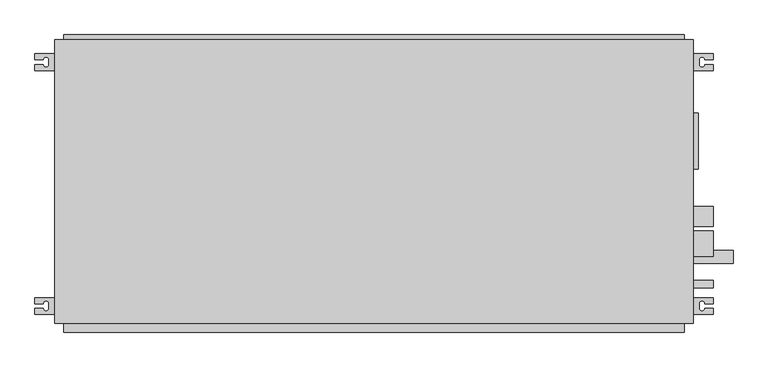
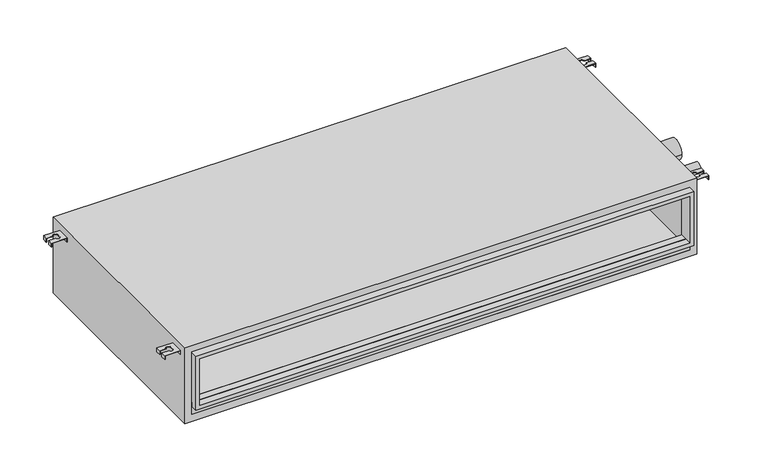
"""IFC4 building model written with IfcOpenShell, lengths in millimetres: proxy geometry, PEFY-P-NMAU-E_Medium_Static_Ducted : PEFY-P54NMAU-E."""

import ifcopenshell
import ifcopenshell.guid

model = None  # the IFC model being written
_history = None  # IfcOwnerHistory: only IFC2X3 demands one
_inside = {}  # id of a spatial element -> (the spatial element, [elements in it])
_under = {}  # id of a project, library or spatial element -> (it, [spatial elements below it])
_declared = {}  # id of a project -> (the project, [libraries it declares])
_typed = {}  # id of a type object -> (the type object, [elements of that type])
_made_of = {}  # id of a material, layer set ... -> (it, [elements and type objects made of it])


def new_model(schema):
    """Start an empty IFC model of exactly this schema.

    Asked for "IFC4X3", IfcOpenShell would pick the latest addendum, in which some entities
    have other attributes; the version numbers below select the first issue.
    IFC2X3 requires an IfcOwnerHistory on every rooted entity: one is made here for all.
    """
    global model, _history
    if schema == "IFC4X3":
        model = ifcopenshell.file(schema_version=(4, 3, 0, 0))
    else:
        model = ifcopenshell.file(schema=schema)
    _inside.clear()
    _under.clear()
    _declared.clear()
    _typed.clear()
    _made_of.clear()
    _history = None
    if model.schema == "IFC2X3":
        org = make("IfcOrganization", Name="unknown")
        user = make(
            "IfcPersonAndOrganization",
            ThePerson=make("IfcPerson", FamilyName="unknown"),
            TheOrganization=org,
        )
        app = make(
            "IfcApplication",
            ApplicationDeveloper=org,
            Version="unknown",
            ApplicationFullName="unknown",
            ApplicationIdentifier="unknown",
        )
        _history = make(
            "IfcOwnerHistory",
            OwningUser=user,
            OwningApplication=app,
            ChangeAction="ADDED",
            CreationDate=0,
        )
    return model


def make(cls, **values):
    """One entity of the class cls with the attributes given. An attribute that is None is left unset."""
    return model.create_entity(
        cls, **{name: value for name, value in values.items() if value is not None}
    )


def rooted(cls, **values):
    """An entity with a GlobalId (a new one), such as an element, a storey or a relation."""
    return make(cls, GlobalId=ifcopenshell.guid.new(), OwnerHistory=_history, **values)


def si_unit(unit_type, name, prefix=None):
    """IfcSIUnit, for example si_unit("LENGTHUNIT", "METRE", prefix="MILLI")."""
    return make("IfcSIUnit", UnitType=unit_type, Prefix=prefix, Name=name)


def assignment(units):
    """IfcUnitAssignment: the units of a project."""
    return None if units is None else make("IfcUnitAssignment", Units=units)


def point(xyz):
    """IfcCartesianPoint."""
    return None if xyz is None else make("IfcCartesianPoint", Coordinates=xyz)


def direction(xyz):
    """IfcDirection."""
    return None if xyz is None else make("IfcDirection", DirectionRatios=xyz)


def frame(location, z_axis=None, x_axis=None):
    """IfcAxis2Placement3D, a coordinate frame: its origin and axes. An axis left out is left unset."""
    return make(
        "IfcAxis2Placement3D",
        Location=point(location),
        Axis=direction(z_axis),
        RefDirection=direction(x_axis),
    )


def frame_2d(location, x_axis=None):
    """IfcAxis2Placement2D, a coordinate frame in the plane: its origin and x axis."""
    return make(
        "IfcAxis2Placement2D", Location=point(location), RefDirection=direction(x_axis)
    )


def origin():
    """The frame at (0, 0, 0) with its axes left unset."""
    return frame((0.0, 0.0, 0.0))


def place(relative_to, where):
    """IfcLocalPlacement: puts the frame where relative to a parent placement (None: the world)."""
    return make(
        "IfcLocalPlacement", PlacementRelTo=relative_to, RelativePlacement=where
    )


def context(
    kind, dimensions, precision=None, world=None, true_north=None, identifier=None
):
    """IfcGeometricRepresentationContext, for example the 3D "Model" context."""
    return make(
        "IfcGeometricRepresentationContext",
        ContextIdentifier=identifier,
        ContextType=kind,
        CoordinateSpaceDimension=dimensions,
        Precision=precision,
        WorldCoordinateSystem=world,
        TrueNorth=true_north,
    )


def project(units=None, contexts=None):
    """IfcProject with its units and contexts."""
    return rooted(
        "IfcProject",
        Name="project",
        RepresentationContexts=contexts,
        UnitsInContext=assignment(units),
    )


def spatial(cls, under=None, at=None, **own):
    """A site, building, storey or space (cls), placed at a placement, below another one or the project."""
    s = rooted(cls, ObjectPlacement=at, **own)
    if under is not None:
        _under.setdefault(under.id(), (under, []))[1].append(s)
    return s


def polyline(points):
    """IfcPolyline through the points."""
    return make("IfcPolyline", Points=[point(p) for p in points])


def circle_curve(where, radius):
    """IfcCircle in the frame where."""
    return make("IfcCircle", Position=where, Radius=radius)


def trimmed(basis, trim1, trim2, sense, master):
    """IfcTrimmedCurve: the piece of a basis curve between two trims."""
    return make(
        "IfcTrimmedCurve",
        BasisCurve=basis,
        Trim1=trim1,
        Trim2=trim2,
        SenseAgreement=sense,
        MasterRepresentation=master,
    )


def segment(curve, same_sense, transition):
    """IfcCompositeCurveSegment."""
    return make(
        "IfcCompositeCurveSegment",
        Transition=transition,
        SameSense=same_sense,
        ParentCurve=curve,
    )


def composite_curve(segments, self_intersect=None):
    """IfcCompositeCurve: segments joined end to end."""
    return make("IfcCompositeCurve", Segments=segments, SelfIntersect=self_intersect)


def outline(outer, holes=None, kind="AREA"):
    """IfcArbitraryClosedProfileDef: a profile drawn as a closed curve; with holes, ...WithVoids."""
    if holes is None:
        return make("IfcArbitraryClosedProfileDef", ProfileType=kind, OuterCurve=outer)
    return make(
        "IfcArbitraryProfileDefWithVoids",
        ProfileType=kind,
        OuterCurve=outer,
        InnerCurves=holes,
    )


def extrude(swept, where, along, depth):
    """IfcExtrudedAreaSolid: the profile swept, set in the frame where, extruded along a direction by depth."""
    return make(
        "IfcExtrudedAreaSolid",
        SweptArea=swept,
        Position=where,
        ExtrudedDirection=direction(along),
        Depth=depth,
    )


def shape(context_of_items, identifier, shape_type, items):
    """IfcShapeRepresentation: the items that make up one representation, for example the "Body"."""
    return make(
        "IfcShapeRepresentation",
        ContextOfItems=context_of_items,
        RepresentationIdentifier=identifier,
        RepresentationType=shape_type,
        Items=items,
    )


def source(mapping_origin, context_of_items, identifier, shape_type, items):
    """IfcRepresentationMap: a shape defined once, which mapped items show again and again."""
    return make(
        "IfcRepresentationMap",
        MappingOrigin=mapping_origin,
        MappedRepresentation=shape(context_of_items, identifier, shape_type, items),
    )


def transform(
    local_origin,
    x_axis=None,
    y_axis=None,
    z_axis=None,
    scale=None,
    scale2=None,
    scale3=None,
    uniform=True,
):
    """IfcCartesianTransformationOperator3D, or its non-uniform kind. x_axis, y_axis, z_axis: its Axis1, 2, 3."""
    if uniform:
        return make(
            "IfcCartesianTransformationOperator3D",
            Axis1=direction(x_axis),
            Axis2=direction(y_axis),
            LocalOrigin=point(local_origin),
            Scale=scale,
            Axis3=direction(z_axis),
        )
    return make(
        "IfcCartesianTransformationOperator3DnonUniform",
        Axis1=direction(x_axis),
        Axis2=direction(y_axis),
        LocalOrigin=point(local_origin),
        Scale=scale,
        Axis3=direction(z_axis),
        Scale2=scale2,
        Scale3=scale3,
    )


def mapped(mapping_source, mapping_target):
    """IfcMappedItem: shows the shape of a source again, moved by a transform."""
    return make(
        "IfcMappedItem", MappingSource=mapping_source, MappingTarget=mapping_target
    )


def made_of(thing, what):
    """Note that an element or type object is made of a material, layer set ...; save() writes the relation."""
    if what is not None:
        _made_of.setdefault(what.id(), (what, []))[1].append(thing)
    return thing


def element(
    cls,
    number,
    at=None,
    inside=None,
    cuts=None,
    type_object=None,
    material=None,
    context=None,
    identifier="Body",
    shape_type=None,
    held_by="IfcProductDefinitionShape",
    body=None,
    shapes=None,
    **own,
):
    """One element of the class cls, such as IfcWall. Its Tag is "e" and its number.

    at: its placement. inside: the storey or other place that contains it. cuts: it is an
    opening in that element (IfcRelVoidsElement). A single representation is given by context,
    identifier, shape_type and body (its items); several are given by shapes. held_by: the class
    of the entity that holds the representations. save() writes the other relations.
    """
    e = rooted(cls, Tag="e%d" % number, ObjectPlacement=at, **own)
    if body is not None:
        shapes = [shape(context, identifier, shape_type, body)]
    if shapes is not None:
        e.Representation = make(held_by, Representations=shapes)
    if inside is not None:
        _inside.setdefault(inside.id(), (inside, []))[1].append(e)
    if cuts is not None:
        rooted(
            "IfcRelVoidsElement", RelatingBuildingElement=cuts, RelatedOpeningElement=e
        )
    if type_object is not None:
        _typed.setdefault(type_object.id(), (type_object, []))[1].append(e)
    return made_of(e, material)


def aggregate(whole, parts):
    """IfcRelAggregates: a whole, such as a stair, and the parts it consists of."""
    return rooted("IfcRelAggregates", RelatingObject=whole, RelatedObjects=parts)


def save(model, path):
    """Write the relations noted so far, then the file.

    IfcRelAggregates (storeys below a building ...), IfcRelContainedInSpatialStructure (elements
    in a storey), IfcRelDefinesByType, IfcRelAssociatesMaterial and IfcRelDeclares: one each for
    every whole, place, type object, material and project.
    """
    for whole, parts in _under.values():
        aggregate(whole, parts)
    for where, things in _inside.values():
        rooted(
            "IfcRelContainedInSpatialStructure",
            RelatedElements=things,
            RelatingStructure=where,
        )
    for kind, things in _typed.values():
        rooted("IfcRelDefinesByType", RelatedObjects=things, RelatingType=kind)
    for what, things in _made_of.values():
        rooted("IfcRelAssociatesMaterial", RelatedObjects=things, RelatingMaterial=what)
    for by, libraries in _declared.values():
        rooted("IfcRelDeclares", RelatingContext=by, RelatedDefinitions=libraries)
    model.write(path)


def plane_surface(at):
    """IfcPlane: the flat surface through the origin of the frame at, square to its z axis."""
    return make("IfcPlane", Position=at)


def revolved_surface(curve, axis_point, axis_direction):
    """IfcSurfaceOfRevolution: the curve turned about the line through axis_point along axis_direction."""
    return make(
        "IfcSurfaceOfRevolution",
        SweptCurve=make("IfcArbitraryOpenProfileDef", ProfileType="CURVE", Curve=curve),
        AxisPosition=make("IfcAxis1Placement", Location=point(axis_point), Axis=direction(axis_direction)),
    )


def advanced_brep(points, edges, surfaces, faces):
    """IfcAdvancedBrep: a solid bounded by faces that lie on surfaces and meet in shared edges.

    An edge is (start, end): straight between two places in points (the first is 0);
    or (start, end, curve); or (start, end, curve, False) where it runs against its curve.
    A face is (place in surfaces, loops), or (place, loops, False) where it looks against
    its surface's normal. A loop lists edges by number (the first is 1), with a minus sign
    where the edge is run from its end to its start. The first loop is the outer one.
    """
    corners = [point(p) for p in points]
    vertices = [make("IfcVertexPoint", VertexGeometry=c) for c in corners]
    made = []
    for start, end, *more in edges:
        made.append(
            make(
                "IfcEdgeCurve",
                EdgeStart=vertices[start],
                EdgeEnd=vertices[end],
                EdgeGeometry=more[0] if more else make("IfcPolyline", Points=[corners[start], corners[end]]),
                SameSense=more[1] if len(more) > 1 else True,
            )
        )
    hull = []
    for where, loops, *sense in faces:
        bounds = []
        for j, loop in enumerate(loops):
            ring = [make("IfcOrientedEdge", EdgeElement=made[abs(k) - 1], Orientation=k > 0) for k in loop]
            bounds.append(
                make(
                    "IfcFaceOuterBound" if j == 0 else "IfcFaceBound",
                    Bound=make("IfcEdgeLoop", EdgeList=ring),
                    Orientation=True,
                )
            )
        hull.append(make("IfcAdvancedFace", Bounds=bounds, FaceSurface=surfaces[where], SameSense=sense[0] if sense else True))
    return make("IfcAdvancedBrep", Outer=make("IfcClosedShell", CfsFaces=hull))


def mechanical_equipment_8a2286fb(model_context):
    return source(origin(), model_context, "Body", "SolidModel", [
        advanced_brep(
        [(-860.118493, -231.05, 249.2375), (-860.118493, -246.05, 249.2375), (-839.112243, -246.05, 249.2375), (-825.112243, -246.05, 249.2375), (-825.112243, -258.05, 249.2375), (-839.112243, -258.05, 249.2375), (-860.118493, -258.05, 249.2375), (-860.118493, -273.05, 249.2375), (-810.112243, -273.05, 249.2375), (-810.112243, -231.05, 249.2375), (-860.118493, -231.05, 236.4972162), (-858.530493, -231.05, 236.4972162), (-858.530493, -246.05, 236.4972162), (-860.118493, -246.05, 236.4972162), (-858.530493, -273.05, 236.4972162), (-860.118493, -273.05, 236.4972162), (-860.118493, -258.05, 236.4972162), (-858.530493, -258.05, 236.4972162), (-810.112243, -231.05, 236.4972162), (-810.112243, -273.05, 236.4972162), (-811.700243, -273.05, 236.4972162), (-811.700243, -231.05, 236.4972162), (-858.530493, -246.05, 247.65), (-839.112243, -246.05, 247.65), (-858.530493, -231.05, 247.65), (-811.700243, -231.05, 247.65), (-858.530493, -258.05, 247.65), (-858.530493, -273.05, 247.65), (-839.112243, -258.05, 247.65), (-811.700243, -273.05, 247.65), (-825.112243, -258.05, 247.65), (-825.112243, -246.05, 247.65)],
        [
            (0, 1),
            (1, 2),
            (2, 3, circle_curve(frame((-832.112243, -246.05, 249.2375), z_axis=(0.0, 0.0, -1.0), x_axis=(1.0, 0.0, 0.0)), 7.0)),
            (3, 4),
            (4, 5, circle_curve(frame((-832.112243, -258.05, 249.2375), z_axis=(0.0, 0.0, -1.0), x_axis=(1.0, 0.0, 0.0)), 7.0)),
            (5, 6),
            (6, 7),
            (7, 8),
            (8, 9),
            (9, 0),
            (10, 11),
            (11, 12),
            (12, 13),
            (13, 10),
            (14, 15),
            (15, 16),
            (16, 17),
            (17, 14),
            (18, 19),
            (19, 20),
            (20, 21),
            (21, 18),
            (13, 1),
            (0, 10),
            (12, 22),
            (22, 23),
            (23, 2),
            (11, 24),
            (24, 22),
            (9, 18),
            (21, 25),
            (25, 24),
            (17, 26),
            (26, 27),
            (27, 14),
            (5, 28),
            (28, 26),
            (16, 6),
            (15, 7),
            (27, 29),
            (29, 20),
            (19, 8),
            (29, 25),
            (30, 31),
            (31, 23, circle_curve(frame((-832.112243, -246.05, 247.65), z_axis=(0.0, 0.0, 1.0), x_axis=(1.0, 0.0, 0.0)), 7.0)),
            (28, 30, circle_curve(frame((-832.112243, -258.05, 247.65), z_axis=(0.0, 0.0, 1.0), x_axis=(1.0, 0.0, 0.0)), 7.0)),
            (4, 30),
            (31, 3),
        ],
        [
            plane_surface(frame((-860.118493, -231.05, 249.2375), z_axis=(0.0, 0.0, 1.0), x_axis=(0.0, -1.0, 0.0))),
            plane_surface(frame((-860.118493, -231.05, 236.4972162), z_axis=(0.0, 0.0, -1.0), x_axis=(0.0, 1.0, 0.0))),
            plane_surface(frame((-860.118493, -231.05, 249.2375), z_axis=(-1.0, 0.0, 0.0), x_axis=(0.0, 0.0, -1.0))),
            plane_surface(frame((-860.118493, -246.05, 249.2375), z_axis=(0.0, -1.0, 0.0), x_axis=(0.0, 0.0, -1.0))),
            plane_surface(frame((-858.530493, -246.05, 249.2375), z_axis=(1.0, 0.0, 0.0), x_axis=(0.0, 0.0, -1.0))),
            plane_surface(frame((-858.530493, -231.05, 249.2375), z_axis=(0.0, 1.0, 0.0), x_axis=(0.0, 0.0, -1.0))),
            plane_surface(frame((-858.530493, -273.05, 249.2375), z_axis=(1.0, 0.0, 0.0), x_axis=(0.0, 0.0, -1.0))),
            plane_surface(frame((-858.530493, -258.05, 249.2375), z_axis=(0.0, 1.0, 0.0), x_axis=(0.0, 0.0, -1.0))),
            plane_surface(frame((-860.118493, -258.05, 249.2375), z_axis=(-1.0, 0.0, 0.0), x_axis=(0.0, 0.0, -1.0))),
            plane_surface(frame((-860.118493, -273.05, 249.2375), z_axis=(0.0, -1.0, 0.0), x_axis=(0.0, 0.0, -1.0))),
            plane_surface(frame((-811.700243, -231.05, 249.2375), z_axis=(-1.0, 0.0, 0.0), x_axis=(0.0, 0.0, -1.0))),
            plane_surface(frame((-810.112243, -273.05, 249.2375), z_axis=(1.0, 0.0, 0.0), x_axis=(0.0, 0.0, -1.0))),
            plane_surface(frame((-825.112243, -258.05, 247.65), z_axis=(0.0, 0.0, -1.0), x_axis=(0.0, 1.0, 0.0))),
            revolved_surface(polyline([(-825.112243, -258.05, 247.65), (-825.112243, -258.05, 249.2375)]), (-832.112243, -258.05, 247.65), (0.0, 0.0, -1.0)),
            revolved_surface(polyline([(-825.112243, -246.05, 247.65), (-825.112243, -246.05, 249.2375)]), (-832.112243, -246.05, 247.65), (0.0, 0.0, -1.0)),
            plane_surface(frame((-825.112243, -246.05, 249.2375), z_axis=(-1.0, 0.0, 0.0), x_axis=(0.0, 0.0, -1.0))),
        ],
        [
            (0, [[1, 2, 3, 4, 5, 6, 7, 8, 9, 10]]),
            (1, [[11, 12, 13, 14]]),
            (1, [[15, 16, 17, 18]]),
            (1, [[19, 20, 21, 22]]),
            (2, [[23, -1, 24, -14]]),
            (3, [[-2, -23, -13, 25, 26, 27]]),
            (4, [[-12, 28, 29, -25]]),
            (5, [[-10, 30, -22, 31, 32, -28, -11, -24]]),
            (6, [[-18, 33, 34, 35]]),
            (7, [[-6, 36, 37, -33, -17, 38]]),
            (8, [[39, -7, -38, -16]]),
            (9, [[-8, -39, -15, -35, 40, 41, -20, 42]]),
            (10, [[-21, -41, 43, -31]]),
            (11, [[-30, -9, -42, -19]]),
            (12, [[44, 45, -26, -29, -32, -43, -40, -34, -37, 46]]),
            (13, [[-5, 47, -46, -36]]),
            (14, [[-3, -27, -45, 48]]),
            (15, [[-4, -48, -44, -47]]),
        ],
    ),
        advanced_brep(
        [(840.094007, -231.05, 249.2375), (790.087757, -231.05, 249.2375), (790.087757, -273.05, 249.2375), (840.094007, -273.05, 249.2375), (840.094007, -258.05, 249.2375), (819.087757, -258.05, 249.2375), (805.087757, -258.05, 249.2375), (805.087757, -246.05, 249.2375), (819.087757, -246.05, 249.2375), (840.094007, -246.05, 249.2375), (840.094007, -231.05, 236.4972162), (840.094007, -246.05, 236.4972162), (838.506007, -246.05, 236.4972162), (838.506007, -231.05, 236.4972162), (838.506007, -273.05, 236.4972162), (838.506007, -258.05, 236.4972162), (840.094007, -258.05, 236.4972162), (840.094007, -273.05, 236.4972162), (790.087757, -231.05, 236.4972162), (791.675757, -231.05, 236.4972162), (791.675757, -273.05, 236.4972162), (790.087757, -273.05, 236.4972162), (819.087757, -246.05, 247.65), (838.506007, -246.05, 247.65), (838.506007, -231.05, 247.65), (791.675757, -231.05, 247.65), (838.506007, -273.05, 247.65), (838.506007, -258.05, 247.65), (819.087757, -258.05, 247.65), (791.675757, -273.05, 247.65), (805.087757, -258.05, 247.65), (805.087757, -246.05, 247.65)],
        [
            (0, 1),
            (1, 2),
            (2, 3),
            (3, 4),
            (4, 5),
            (5, 6, circle_curve(frame((812.087757, -258.05, 249.2375), z_axis=(0.0, 0.0, -1.0), x_axis=(-1.0, 0.0, 0.0)), 7.0)),
            (6, 7),
            (7, 8, circle_curve(frame((812.087757, -246.05, 249.2375), z_axis=(0.0, 0.0, -1.0), x_axis=(-1.0, 0.0, 0.0)), 7.0)),
            (8, 9),
            (9, 0),
            (10, 11),
            (11, 12),
            (12, 13),
            (13, 10),
            (14, 15),
            (15, 16),
            (16, 17),
            (17, 14),
            (18, 19),
            (19, 20),
            (20, 21),
            (21, 18),
            (10, 0),
            (9, 11),
            (8, 22),
            (22, 23),
            (23, 12),
            (23, 24),
            (24, 13),
            (24, 25),
            (25, 19),
            (18, 1),
            (14, 26),
            (26, 27),
            (27, 15),
            (4, 16),
            (27, 28),
            (28, 5),
            (3, 17),
            (2, 21),
            (20, 29),
            (29, 26),
            (25, 29),
            (30, 28, circle_curve(frame((812.087757, -258.05, 247.65), z_axis=(0.0, 0.0, 1.0), x_axis=(-1.0, 0.0, 0.0)), 7.0)),
            (22, 31, circle_curve(frame((812.087757, -246.05, 247.65), z_axis=(0.0, 0.0, 1.0), x_axis=(-1.0, 0.0, 0.0)), 7.0)),
            (31, 30),
            (30, 6),
            (7, 31),
        ],
        [
            plane_surface(frame((840.094007, -231.05, 249.2375), z_axis=(0.0, 0.0, 1.0), x_axis=(0.0, -1.0, 0.0))),
            plane_surface(frame((840.094007, -231.05, 236.4972162), z_axis=(0.0, 0.0, -1.0), x_axis=(0.0, 1.0, 0.0))),
            plane_surface(frame((840.094007, -231.05, 249.2375), z_axis=(1.0, 0.0, 0.0), x_axis=(0.0, 0.0, -1.0))),
            plane_surface(frame((840.094007, -246.05, 249.2375), z_axis=(0.0, -1.0, 0.0), x_axis=(0.0, 0.0, -1.0))),
            plane_surface(frame((838.506007, -246.05, 249.2375), z_axis=(-1.0, 0.0, 0.0), x_axis=(0.0, 0.0, -1.0))),
            plane_surface(frame((838.506007, -231.05, 249.2375), z_axis=(0.0, 1.0, 0.0), x_axis=(0.0, 0.0, -1.0))),
            plane_surface(frame((838.506007, -273.05, 249.2375), z_axis=(-1.0, 0.0, 0.0), x_axis=(0.0, 0.0, -1.0))),
            plane_surface(frame((838.506007, -258.05, 249.2375), z_axis=(0.0, 1.0, 0.0), x_axis=(0.0, 0.0, -1.0))),
            plane_surface(frame((840.094007, -258.05, 249.2375), z_axis=(1.0, 0.0, 0.0), x_axis=(0.0, 0.0, -1.0))),
            plane_surface(frame((840.094007, -273.05, 249.2375), z_axis=(0.0, -1.0, 0.0), x_axis=(0.0, 0.0, -1.0))),
            plane_surface(frame((791.675757, -231.05, 249.2375), z_axis=(1.0, 0.0, 0.0), x_axis=(0.0, 0.0, -1.0))),
            plane_surface(frame((790.087757, -273.05, 249.2375), z_axis=(-1.0, 0.0, 0.0), x_axis=(0.0, 0.0, -1.0))),
            plane_surface(frame((805.087757, -258.05, 247.65), z_axis=(0.0, 0.0, -1.0), x_axis=(0.0, 1.0, 0.0))),
            revolved_surface(polyline([(805.087757, -258.05, 247.65), (805.087757, -258.05, 249.2375)]), (812.087757, -258.05, 247.65), (0.0, 0.0, -1.0)),
            revolved_surface(polyline([(805.087757, -246.05, 247.65), (805.087757, -246.05, 249.2375)]), (812.087757, -246.05, 247.65), (0.0, 0.0, -1.0)),
            plane_surface(frame((805.087757, -246.05, 249.2375), z_axis=(1.0, 0.0, 0.0), x_axis=(0.0, 0.0, -1.0))),
        ],
        [
            (0, [[1, 2, 3, 4, 5, 6, 7, 8, 9, 10]]),
            (1, [[11, 12, 13, 14]]),
            (1, [[15, 16, 17, 18]]),
            (1, [[19, 20, 21, 22]]),
            (2, [[-11, 23, -10, 24]]),
            (3, [[25, 26, 27, -12, -24, -9]]),
            (4, [[-27, 28, 29, -13]]),
            (5, [[-23, -14, -29, 30, 31, -19, 32, -1]]),
            (6, [[33, 34, 35, -15]]),
            (7, [[36, -16, -35, 37, 38, -5]]),
            (8, [[-17, -36, -4, 39]]),
            (9, [[40, -21, 41, 42, -33, -18, -39, -3]]),
            (10, [[-31, 43, -41, -20]]),
            (11, [[-22, -40, -2, -32]]),
            (12, [[44, -37, -34, -42, -43, -30, -28, -26, 45, 46]]),
            (13, [[-38, -44, 47, -6]]),
            (14, [[48, -45, -25, -8]]),
            (15, [[-47, -46, -48, -7]]),
        ],
    ),
        advanced_brep(
        [(-860.118493, 339.0, 249.2375), (-810.112243, 339.0, 249.2375), (-810.112243, 381.0, 249.2375), (-860.118493, 381.0, 249.2375), (-860.118493, 366.0, 249.2375), (-839.112243, 366.0, 249.2375), (-825.112243, 366.0, 249.2375), (-825.112243, 354.0, 249.2375), (-839.112243, 354.0, 249.2375), (-860.118493, 354.0, 249.2375), (-860.118493, 339.0, 236.4972162), (-860.118493, 354.0, 236.4972162), (-858.530493, 354.0, 236.4972162), (-858.530493, 339.0, 236.4972162), (-858.530493, 381.0, 236.4972162), (-858.530493, 366.0, 236.4972162), (-860.118493, 366.0, 236.4972162), (-860.118493, 381.0, 236.4972162), (-810.112243, 339.0, 236.4972162), (-811.700243, 339.0, 236.4972162), (-811.700243, 381.0, 236.4972162), (-810.112243, 381.0, 236.4972162), (-839.112243, 354.0, 247.65), (-858.530493, 354.0, 247.65), (-858.530493, 339.0, 247.65), (-811.700243, 339.0, 247.65), (-858.530493, 381.0, 247.65), (-858.530493, 366.0, 247.65), (-839.112243, 366.0, 247.65), (-811.700243, 381.0, 247.65), (-825.112243, 366.0, 247.65), (-825.112243, 354.0, 247.65)],
        [
            (0, 1),
            (1, 2),
            (2, 3),
            (3, 4),
            (4, 5),
            (5, 6, circle_curve(frame((-832.112243, 366.0, 249.2375), z_axis=(0.0, 0.0, -1.0), x_axis=(1.0, 0.0, 0.0)), 7.0)),
            (6, 7),
            (7, 8, circle_curve(frame((-832.112243, 354.0, 249.2375), z_axis=(0.0, 0.0, -1.0), x_axis=(1.0, 0.0, 0.0)), 7.0)),
            (8, 9),
            (9, 0),
            (10, 11),
            (11, 12),
            (12, 13),
            (13, 10),
            (14, 15),
            (15, 16),
            (16, 17),
            (17, 14),
            (18, 19),
            (19, 20),
            (20, 21),
            (21, 18),
            (10, 0),
            (9, 11),
            (8, 22),
            (22, 23),
            (23, 12),
            (23, 24),
            (24, 13),
            (24, 25),
            (25, 19),
            (18, 1),
            (14, 26),
            (26, 27),
            (27, 15),
            (4, 16),
            (27, 28),
            (28, 5),
            (3, 17),
            (2, 21),
            (20, 29),
            (29, 26),
            (25, 29),
            (30, 28, circle_curve(frame((-832.112243, 366.0, 247.65), z_axis=(0.0, 0.0, 1.0), x_axis=(1.0, 0.0, 0.0)), 7.0)),
            (22, 31, circle_curve(frame((-832.112243, 354.0, 247.65), z_axis=(0.0, 0.0, 1.0), x_axis=(1.0, 0.0, 0.0)), 7.0)),
            (31, 30),
            (30, 6),
            (7, 31),
        ],
        [
            plane_surface(frame((-860.118493, 339.0, 249.2375), z_axis=(0.0, 0.0, 1.0), x_axis=(0.0, 1.0, 0.0))),
            plane_surface(frame((-860.118493, 339.0, 236.4972162), z_axis=(0.0, 0.0, -1.0), x_axis=(0.0, -1.0, 0.0))),
            plane_surface(frame((-860.118493, 339.0, 249.2375), z_axis=(-1.0, 0.0, 0.0), x_axis=(0.0, 0.0, -1.0))),
            plane_surface(frame((-860.118493, 354.0, 249.2375), z_axis=(0.0, 1.0, 0.0), x_axis=(0.0, 0.0, -1.0))),
            plane_surface(frame((-858.530493, 354.0, 249.2375), z_axis=(1.0, 0.0, 0.0), x_axis=(0.0, 0.0, -1.0))),
            plane_surface(frame((-858.530493, 339.0, 249.2375), z_axis=(0.0, -1.0, 0.0), x_axis=(0.0, 0.0, -1.0))),
            plane_surface(frame((-858.530493, 381.0, 249.2375), z_axis=(1.0, 0.0, 0.0), x_axis=(0.0, 0.0, -1.0))),
            plane_surface(frame((-858.530493, 366.0, 249.2375), z_axis=(0.0, -1.0, 0.0), x_axis=(0.0, 0.0, -1.0))),
            plane_surface(frame((-860.118493, 366.0, 249.2375), z_axis=(-1.0, 0.0, 0.0), x_axis=(0.0, 0.0, -1.0))),
            plane_surface(frame((-860.118493, 381.0, 249.2375), z_axis=(0.0, 1.0, 0.0), x_axis=(0.0, 0.0, -1.0))),
            plane_surface(frame((-811.700243, 339.0, 249.2375), z_axis=(-1.0, 0.0, 0.0), x_axis=(0.0, 0.0, -1.0))),
            plane_surface(frame((-810.112243, 381.0, 249.2375), z_axis=(1.0, 0.0, 0.0), x_axis=(0.0, 0.0, -1.0))),
            plane_surface(frame((-825.112243, 366.0, 247.65), z_axis=(0.0, 0.0, -1.0), x_axis=(0.0, -1.0, 0.0))),
            revolved_surface(polyline([(-825.112243, 366.0, 247.65), (-825.112243, 366.0, 249.2375)]), (-832.112243, 366.0, 247.65), (0.0, 0.0, -1.0)),
            revolved_surface(polyline([(-825.112243, 354.0, 247.65), (-825.112243, 354.0, 249.2375)]), (-832.112243, 354.0, 247.65), (0.0, 0.0, -1.0)),
            plane_surface(frame((-825.112243, 354.0, 249.2375), z_axis=(-1.0, 0.0, 0.0), x_axis=(0.0, 0.0, -1.0))),
        ],
        [
            (0, [[1, 2, 3, 4, 5, 6, 7, 8, 9, 10]]),
            (1, [[11, 12, 13, 14]]),
            (1, [[15, 16, 17, 18]]),
            (1, [[19, 20, 21, 22]]),
            (2, [[-11, 23, -10, 24]]),
            (3, [[25, 26, 27, -12, -24, -9]]),
            (4, [[-27, 28, 29, -13]]),
            (5, [[-23, -14, -29, 30, 31, -19, 32, -1]]),
            (6, [[33, 34, 35, -15]]),
            (7, [[36, -16, -35, 37, 38, -5]]),
            (8, [[-17, -36, -4, 39]]),
            (9, [[40, -21, 41, 42, -33, -18, -39, -3]]),
            (10, [[-31, 43, -41, -20]]),
            (11, [[-22, -40, -2, -32]]),
            (12, [[44, -37, -34, -42, -43, -30, -28, -26, 45, 46]]),
            (13, [[-38, -44, 47, -6]]),
            (14, [[48, -45, -25, -8]]),
            (15, [[-47, -46, -48, -7]]),
        ],
    ),
        advanced_brep(
        [(840.094007, 339.0, 249.2375), (840.094007, 354.0, 249.2375), (819.087757, 354.0, 249.2375), (805.087757, 354.0, 249.2375), (805.087757, 366.0, 249.2375), (819.087757, 366.0, 249.2375), (840.094007, 366.0, 249.2375), (840.094007, 381.0, 249.2375), (790.087757, 381.0, 249.2375), (790.087757, 339.0, 249.2375), (840.094007, 339.0, 236.4972162), (838.506007, 339.0, 236.4972162), (838.506007, 354.0, 236.4972162), (840.094007, 354.0, 236.4972162), (838.506007, 381.0, 236.4972162), (840.094007, 381.0, 236.4972162), (840.094007, 366.0, 236.4972162), (838.506007, 366.0, 236.4972162), (790.087757, 339.0, 236.4972162), (790.087757, 381.0, 236.4972162), (791.675757, 381.0, 236.4972162), (791.675757, 339.0, 236.4972162), (838.506007, 354.0, 247.65), (819.087757, 354.0, 247.65), (838.506007, 339.0, 247.65), (791.675757, 339.0, 247.65), (838.506007, 366.0, 247.65), (838.506007, 381.0, 247.65), (819.087757, 366.0, 247.65), (791.675757, 381.0, 247.65), (805.087757, 366.0, 247.65), (805.087757, 354.0, 247.65)],
        [
            (0, 1),
            (1, 2),
            (2, 3, circle_curve(frame((812.087757, 354.0, 249.2375), z_axis=(0.0, 0.0, -1.0), x_axis=(-1.0, 0.0, 0.0)), 7.0)),
            (3, 4),
            (4, 5, circle_curve(frame((812.087757, 366.0, 249.2375), z_axis=(0.0, 0.0, -1.0), x_axis=(-1.0, 0.0, 0.0)), 7.0)),
            (5, 6),
            (6, 7),
            (7, 8),
            (8, 9),
            (9, 0),
            (10, 11),
            (11, 12),
            (12, 13),
            (13, 10),
            (14, 15),
            (15, 16),
            (16, 17),
            (17, 14),
            (18, 19),
            (19, 20),
            (20, 21),
            (21, 18),
            (13, 1),
            (0, 10),
            (12, 22),
            (22, 23),
            (23, 2),
            (11, 24),
            (24, 22),
            (9, 18),
            (21, 25),
            (25, 24),
            (17, 26),
            (26, 27),
            (27, 14),
            (5, 28),
            (28, 26),
            (16, 6),
            (15, 7),
            (27, 29),
            (29, 20),
            (19, 8),
            (29, 25),
            (30, 31),
            (31, 23, circle_curve(frame((812.087757, 354.0, 247.65), z_axis=(0.0, 0.0, 1.0), x_axis=(-1.0, 0.0, 0.0)), 7.0)),
            (28, 30, circle_curve(frame((812.087757, 366.0, 247.65), z_axis=(0.0, 0.0, 1.0), x_axis=(-1.0, 0.0, 0.0)), 7.0)),
            (4, 30),
            (31, 3),
        ],
        [
            plane_surface(frame((840.094007, 339.0, 249.2375), z_axis=(0.0, 0.0, 1.0), x_axis=(0.0, 1.0, 0.0))),
            plane_surface(frame((840.094007, 339.0, 236.4972162), z_axis=(0.0, 0.0, -1.0), x_axis=(0.0, -1.0, 0.0))),
            plane_surface(frame((840.094007, 339.0, 249.2375), z_axis=(1.0, 0.0, 0.0), x_axis=(0.0, 0.0, -1.0))),
            plane_surface(frame((840.094007, 354.0, 249.2375), z_axis=(0.0, 1.0, 0.0), x_axis=(0.0, 0.0, -1.0))),
            plane_surface(frame((838.506007, 354.0, 249.2375), z_axis=(-1.0, 0.0, 0.0), x_axis=(0.0, 0.0, -1.0))),
            plane_surface(frame((838.506007, 339.0, 249.2375), z_axis=(0.0, -1.0, 0.0), x_axis=(0.0, 0.0, -1.0))),
            plane_surface(frame((838.506007, 381.0, 249.2375), z_axis=(-1.0, 0.0, 0.0), x_axis=(0.0, 0.0, -1.0))),
            plane_surface(frame((838.506007, 366.0, 249.2375), z_axis=(0.0, -1.0, 0.0), x_axis=(0.0, 0.0, -1.0))),
            plane_surface(frame((840.094007, 366.0, 249.2375), z_axis=(1.0, 0.0, 0.0), x_axis=(0.0, 0.0, -1.0))),
            plane_surface(frame((840.094007, 381.0, 249.2375), z_axis=(0.0, 1.0, 0.0), x_axis=(0.0, 0.0, -1.0))),
            plane_surface(frame((791.675757, 339.0, 249.2375), z_axis=(1.0, 0.0, 0.0), x_axis=(0.0, 0.0, -1.0))),
            plane_surface(frame((790.087757, 381.0, 249.2375), z_axis=(-1.0, 0.0, 0.0), x_axis=(0.0, 0.0, -1.0))),
            plane_surface(frame((805.087757, 366.0, 247.65), z_axis=(0.0, 0.0, -1.0), x_axis=(0.0, -1.0, 0.0))),
            revolved_surface(polyline([(805.087757, 366.0, 247.65), (805.087757, 366.0, 249.2375)]), (812.087757, 366.0, 247.65), (0.0, 0.0, -1.0)),
            revolved_surface(polyline([(805.087757, 354.0, 247.65), (805.087757, 354.0, 249.2375)]), (812.087757, 354.0, 247.65), (0.0, 0.0, -1.0)),
            plane_surface(frame((805.087757, 354.0, 249.2375), z_axis=(1.0, 0.0, 0.0), x_axis=(0.0, 0.0, -1.0))),
        ],
        [
            (0, [[1, 2, 3, 4, 5, 6, 7, 8, 9, 10]]),
            (1, [[11, 12, 13, 14]]),
            (1, [[15, 16, 17, 18]]),
            (1, [[19, 20, 21, 22]]),
            (2, [[23, -1, 24, -14]]),
            (3, [[-2, -23, -13, 25, 26, 27]]),
            (4, [[-12, 28, 29, -25]]),
            (5, [[-10, 30, -22, 31, 32, -28, -11, -24]]),
            (6, [[-18, 33, 34, 35]]),
            (7, [[-6, 36, 37, -33, -17, 38]]),
            (8, [[39, -7, -38, -16]]),
            (9, [[-8, -39, -15, -35, 40, 41, -20, 42]]),
            (10, [[-21, -41, 43, -31]]),
            (11, [[-30, -9, -42, -19]]),
            (12, [[44, 45, -26, -29, -32, -43, -40, -34, -37, 46]]),
            (13, [[-5, 47, -46, -36]]),
            (14, [[-3, -27, -45, 48]]),
            (15, [[-4, -48, -44, -47]]),
        ],
    ),
        extrude(outline(polyline([(767.862757, -295.275), (-787.887243, -295.275), (-787.887243, -273.05), (767.862757, -273.05), (767.862757, -295.275)])), frame((0.0, 0.0, 42.8625), z_axis=(0.0, 0.0, 1.0), x_axis=(1.0, 0.0, 0.0)), (0.0, 0.0, 1.0), 39.6875),
        extrude(outline(polyline([(249.2375, 767.862757), (249.2375, -787.887243), (69.85, -787.887243), (69.85, 767.862757), (249.2375, 767.862757)]), holes=[polyline([(82.55, 755.162757), (82.55, -775.187243), (236.5375, -775.187243), (236.5375, 755.162757), (82.55, 755.162757)])]), frame((0.0, -317.5, 0.0), z_axis=(0.0, 1.0, 0.0), x_axis=(0.0, 0.0, 1.0)), (0.0, 0.0, 1.0), 44.45),
        extrude(outline(polyline([(767.862757, 415.925), (-787.887243, 415.925), (-787.887243, 428.625), (767.862757, 428.625), (767.862757, 415.925)])), frame((0.0, 0.0, 42.8625), z_axis=(0.0, 0.0, 1.0), x_axis=(1.0, 0.0, 0.0)), (0.0, 0.0, 1.0), 206.375),
        extrude(outline(polyline([(271.4625, 790.087757), (271.4625, -810.112243), (20.6375, -810.112243), (20.6375, 790.087757), (271.4625, 790.087757)]), holes=[polyline([(42.8625, -787.887243), (249.2375, -787.887243), (249.2375, 767.862757), (42.8625, 767.862757), (42.8625, -787.887243)])]), frame((0.0, -295.275, 0.0), z_axis=(0.0, 1.0, 0.0), x_axis=(0.0, 0.0, 1.0)), (0.0, 0.0, 1.0), 711.2),
        extrude(outline(composite_curve([segment(trimmed(circle_curve(frame_2d((-26.9875, 109.5375)), 25.4), [point((-1.5875, 109.5375))], [point((-52.3875, 109.5375))], False, "CARTESIAN"), True, "CONTINUOUS"), segment(trimmed(circle_curve(frame_2d((-26.9875, 109.5375)), 25.4), [point((-52.3875, 109.5375))], [point((-1.5875, 109.5375))], False, "CARTESIAN"), True, "CONTINUOUS")], self_intersect=False)), frame((790.087757, 0.0, 0.0), z_axis=(1.0, 0.0, 0.0), x_axis=(0.0, 1.0, 0.0)), (0.0, 0.0, 1.0), 50.00625),
        extrude(outline(composite_curve([segment(trimmed(circle_curve(frame_2d((-128.5875, 171.45)), 15.875), [point((-112.7125, 171.45))], [point((-144.4625, 171.45))], False, "CARTESIAN"), True, "CONTINUOUS"), segment(trimmed(circle_curve(frame_2d((-128.5875, 171.45)), 15.875), [point((-144.4625, 171.45))], [point((-112.7125, 171.45))], False, "CARTESIAN"), True, "CONTINUOUS")], self_intersect=False)), frame((790.087757, 0.0, 0.0), z_axis=(1.0, 0.0, 0.0), x_axis=(0.0, 1.0, 0.0)), (0.0, 0.0, 1.0), 100.0125),
        extrude(outline(composite_curve([segment(trimmed(circle_curve(frame_2d((-95.25, 230.1875)), 31.75), [point((-63.5, 230.1875))], [point((-127.0, 230.1875))], False, "CARTESIAN"), True, "CONTINUOUS"), segment(trimmed(circle_curve(frame_2d((-95.25, 230.1875)), 31.75), [point((-127.0, 230.1875))], [point((-63.5, 230.1875))], False, "CARTESIAN"), True, "CONTINUOUS")], self_intersect=False)), frame((790.087757, 0.0, 0.0), z_axis=(1.0, 0.0, 0.0), x_axis=(0.0, 1.0, 0.0)), (0.0, 0.0, 1.0), 50.00625),
        extrude(outline(composite_curve([segment(trimmed(circle_curve(frame_2d((-196.85, 104.775)), 9.525), [point((-187.325, 104.775))], [point((-206.375, 104.775))], False, "CARTESIAN"), True, "CONTINUOUS"), segment(trimmed(circle_curve(frame_2d((-196.85, 104.775)), 9.525), [point((-206.375, 104.775))], [point((-187.325, 104.775))], False, "CARTESIAN"), True, "CONTINUOUS")], self_intersect=False)), frame((790.087757, 0.0, 0.0), z_axis=(1.0, 0.0, 0.0), x_axis=(0.0, 1.0, 0.0)), (0.0, 0.0, 1.0), 50.00625),
        extrude(outline(polyline([(802.787757, 231.84375), (802.787757, 92.14375), (790.087757, 92.14375), (790.087757, 231.84375), (802.787757, 231.84375)])), frame((0.0, 0.0, 42.8625), z_axis=(0.0, 0.0, 1.0), x_axis=(1.0, 0.0, 0.0)), (0.0, 0.0, 1.0), 187.325),
    ])


if __name__ == "__main__":
    model = new_model("IFC4")
    model_context = context("Model", 3, world=origin())
    ifc_project = project(units=[si_unit("LENGTHUNIT", "METRE", prefix="MILLI")], contexts=[model_context])
    site = spatial("IfcSite", under=ifc_project)
    building = spatial("IfcBuilding", under=site)
    placement = place(None, origin())
    mechanical_equipment_shape = mechanical_equipment_8a2286fb(model_context)
    element("IfcBuildingElementProxy", 1, Name="PEFY-P-NMAU-E_Medium_Static_Ducted : PEFY-P54NMAU-E", ObjectType="PEFY-P-NMAU-E_Medium_Static_Ducted : PEFY-P54NMAU-E", at=placement, inside=building, context=model_context, shape_type="MappedRepresentation", body=[
        mapped(mechanical_equipment_shape, transform((0.0, 0.0, 0.0), x_axis=(1.0, 0.0, 0.0), y_axis=(0.0, 1.0, 0.0), z_axis=(0.0, 0.0, 1.0))),
    ])
    save(model, "model.ifc")

# Revit data of these elements
# Type "PEFY-P-NMAU-E_Medium_Static_Ducted : PEFY-P54NMAU-E"
#   Wiring (Min.size of wire) = "1/8"
#   Wiring (Amperage of wire breaker) = "15 A"
#   Voltage Options = "208/230 VAC"
#   Unit Weight (LBS) = "102"
#   Temperature set range Remote controller Heating = "63 to 83 F"
#   Temperature set range Remote controller Cooling = "67 to 86 F"
#   Subcategory = "HVAC"
#   Specification URL = ""
#   Sound Pressure Levels (dB(A)) = "26,28,29"
#   SmartBIM Object Created By = "Reed Construction Data"
#   Single Phase = "X"
#   Refrigerant control device = "LEV"
#   Protection devices = "Fuse"
#   Power input Heating = "0.34 kW"
#   Power input Cooling = "0.36 kW"
#   Moter Type = "DC blushless motor"
#   Moter Output = "0.085 kW"
#   Model = "PEFY-P54NMAU-E"
#   Manufacturer URL = ""
#   Manufacturer = "Mitsubishi Electric"
#   Insulation material = "EPS, Polyethylene foam, Urethane foam"
#   Installation URL = ""
#   Heating Capacity (kcal/h) = "15,100"
#   Heating Capacity (kW) = "17.6"
#   Heat exchanger = "Cross fin(Aluminium fin and copper tube)"
#   Frequency = "60 Hz"
#   Fan Type x Quantity = "Sirocco fan x 1"
#   E.S.P(mmH2O) = "3.6,5.1,7.1,10.2,15.3"
#   E.S.P(Pa) = "35,50,70,100,150"
#   E.S.P(In. W.G.) = "0.14,0.20,0.28,0.40,0.60"
#   Driving mechanism = "Direct-driven by motor"
#   Current Heating = "2.13 A"
#   Current Cooling = "2.24 A"
#   Cooling Capacity (kcal/h) = "13,600"
#   Cooling Capacity (kW) = "15.8"
#   Connectable outdoor unit = "R410A,R22 CITY MULTI"
#   Assembly Code = "D3050200"
#   Airflow rate(Low-Mid-High) (m3/min) = "6.0,7.5,8.5"
#   Airflow rate(Low-Mid-High) (cfm) = "212,265,300"
#   Airflow rate(Low-Mid-High) (L/s) = "100,125,142"
#   Air Filter = "PP Honeycomb fabric"
#   95 CSI = "15760"
#   04 CSI = "23 82 19"
#   Width = 5' - 3"
#   Voltage = 208 V
#   Unit Supply Airflow [instance default] = 0 CFM
#   Unit Return Airflow [instance default] = 0 CFM
#   SmartBIM Object Version = 3
#   Refrigerant Pipe Liquid = 0' - 0 3/8"
#   Refrigerant Pipe Gas = 0' - 0 5/8"
#   Refirigerant Pipe diameter (Liquid) = 0' - 0 3/8"
#   Refirigerant Pipe diameter (Gas) = 0' - 0 5/8"
#   Phase = 1
#   Nominal Heating Capacity = 60000.0 Btu/h
#   Nominal Cooling Capacity = 54000.0 Btu/h
#   Minimum Circuit Current = 3.31 A
#   Maximum Overcurrent Protection = 15 A
#   Hertz = 60
#   Height = 0' - 9 7/8"
#   Drain piping diameter = 0' - 1 1/4"
#   Drain Pump = 0' - 1"
#   Depth = 2' - 4 7/8"
#   Default Elevation = 4' - 0"
#   Back Air Inlet Width = 5' - 1 1/4"
#   Back Air Inlet Height = 0' - 8 1/8"
#   Apparent Load = 0 VA
#   Air Outlet Width = 5' - 1 1/4"
#   Air Outlet Height = 0' - 7 1/16"
#   Sound Pressure Levels @ Mid Airflow (dBA) = 41
#   Sound Pressure Levels @ Low Airflow (dBA) = 36
#   Sound Pressure Levels @ High Airflow (dBA) = 45
#   Number of Poles = 2
#   Unit = Metal - Steel Satin
#   Load Classification = Other
#   Back Air Inlet = Grille
# Element 1 (IfcBuildingElementProxy, "PEFY-P-NMAU-E_Medium_Static_Ducted : PEFY-P54NMAU-E")
#   Materials on its faces: "Metal - Steel Satin", "Grille"
# Materials
#   "Metal - Steel Satin": class "Metal", colour RGB 189 187 185, transparency 0
#   "Grille": class "Miscellaneous", colour RGB 0 0 0, transparency 0
